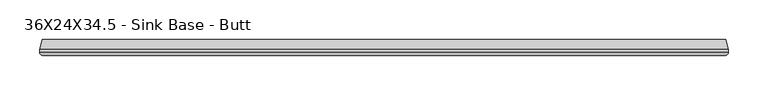
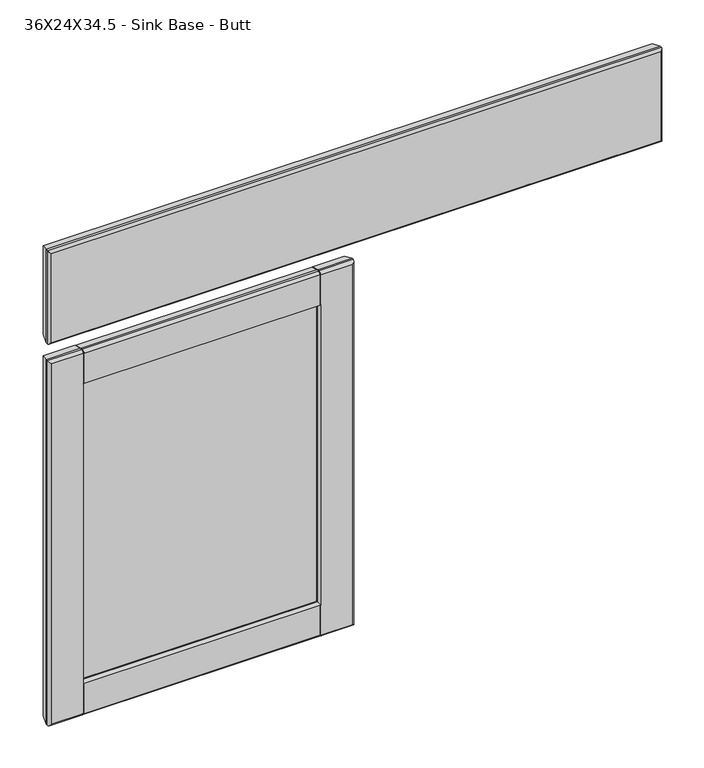
"""IFC4 building model written with IfcOpenShell, lengths in millimetres: furniture geometry, Cabinet-Base-Merillat-Double_Door-Marlin : 36X24X34.5 - Sink Base - Butt."""

from ifc_helpers import new_model, si_unit, frame, origin, place, context, project, spatial, polyline, circle_curve, ellipse_curve, outline, extrude, source, transform, mapped, element, save
from ifc_brep_helpers import plane_surface, cylinder_surface, advanced_brep


def furniture_36x24x34_5_sink_base_butt_1b95edc5(model_context):
    return source(origin(), model_context, "Body", "SolidModel", [
        advanced_brep(
        [(-413.1408026, -629.92, 847.8035075), (-413.1408026, -629.92, 714.2964925), (450.6162124, -629.92, 714.2964925), (450.6162124, -629.92, 847.8035075), (-412.7320951, -609.6, 714.7052), (-412.7320951, -609.6, 847.3948), (450.2075049, -609.6, 847.3948), (450.2075049, -609.6, 714.7052), (-416.2372951, -625.4496, 850.9), (-416.2372951, -622.681, 850.9), (-416.2372951, -622.681, 711.2), (-416.2372951, -625.4496, 711.2), (453.7127049, -622.681, 711.2), (453.7127049, -625.4496, 711.2), (453.7127049, -622.681, 850.9), (453.7127049, -625.4496, 850.9)],
        [
            (0, 1),
            (1, 2),
            (2, 3),
            (3, 0),
            (4, 5),
            (5, 6),
            (6, 7),
            (7, 4),
            (8, 9),
            (9, 10),
            (10, 11),
            (11, 8),
            (10, 12),
            (12, 13),
            (13, 11),
            (12, 14),
            (14, 15),
            (15, 13),
            (8, 15),
            (14, 9),
            (11, 1, ellipse_curve(frame((-411.4620951, -625.4496, 715.9752), z_axis=(-0.7071067811865475, 0.0, 0.7071067811865475), x_axis=(-0.7071067811865474, 0.0, -0.7071067811865476)), 6.7531526, 4.7752)),
            (0, 8, ellipse_curve(frame((-411.4620951, -625.4496, 846.1248), z_axis=(-0.7071067811865475, 0.0, -0.7071067811865475), x_axis=(0.7071067811865474, 0.0, -0.7071067811865476)), 6.7531526, 4.7752)),
            (4, 10),
            (9, 5),
            (13, 2, ellipse_curve(frame((448.9375049, -625.4496, 715.9752), z_axis=(-0.7071067811865475, 0.0, -0.7071067811865475), x_axis=(0.7071067811865476, 0.0, -0.7071067811865474)), 6.7531526, 4.7752)),
            (7, 12),
            (15, 3, ellipse_curve(frame((448.9375049, -625.4496, 846.1248), z_axis=(0.7071067811865475, 0.0, -0.7071067811865475), x_axis=(0.7071067811865474, 0.0, 0.7071067811865476)), 6.7531526, 4.7752)),
            (6, 14),
        ],
        [
            plane_surface(frame((-416.2372951, -629.92, 850.9), z_axis=(0.0, -1.0, 0.0), x_axis=(0.0, 0.0, -1.0))),
            plane_surface(frame((-416.2372951, -609.6, 850.9), z_axis=(0.0, 1.0, 0.0), x_axis=(0.0, 0.0, 1.0))),
            plane_surface(frame((-416.2372951, -629.92, 850.9), z_axis=(-1.0, 0.0, 0.0), x_axis=(0.0, 1.0, 0.0))),
            plane_surface(frame((-416.2372951, -629.92, 711.2), z_axis=(0.0, 0.0, -1.0), x_axis=(0.0, 1.0, 0.0))),
            plane_surface(frame((453.7127049, -629.92, 711.2), z_axis=(1.0, 0.0, 0.0), x_axis=(0.0, 1.0, 0.0))),
            plane_surface(frame((453.7127049, -629.92, 850.9), z_axis=(0.0, 0.0, 1.0), x_axis=(0.0, 1.0, 0.0))),
            cylinder_surface(frame((-411.4620951, -625.4496, 850.9), z_axis=(0.0, 0.0, -1.0), x_axis=(0.0, 1.0, 0.0)), 4.7752),
            plane_surface(frame((-416.2372951, -622.681, 850.9), z_axis=(-0.9659229350723619, 0.25882983502910506, 0.0), x_axis=(0.0, 0.0, -1.0))),
            cylinder_surface(frame((-416.2372951, -625.4496, 715.9752), z_axis=(1.0, 0.0, 0.0), x_axis=(0.0, 1.0, 0.0)), 4.7752),
            plane_surface(frame((-416.2372951, -622.681, 711.2), z_axis=(0.0, 0.25882983502910506, -0.9659229350723619), x_axis=(1.0, 0.0, 0.0))),
            cylinder_surface(frame((448.9375049, -625.4496, 711.2), z_axis=(0.0, 0.0, 1.0), x_axis=(0.0, 1.0, 0.0)), 4.7752),
            plane_surface(frame((453.7127049, -622.681, 711.2), z_axis=(0.9659229350723619, 0.25882983502910506, 0.0), x_axis=(0.0, 0.0, 1.0))),
            cylinder_surface(frame((453.7127049, -625.4496, 846.1248), z_axis=(-1.0, 0.0, 0.0), x_axis=(0.0, 1.0, 0.0)), 4.7752),
            plane_surface(frame((453.7127049, -622.681, 850.9), z_axis=(0.0, 0.25882983502910506, 0.9659229350723619), x_axis=(-1.0, 0.0, 0.0))),
        ],
        [
            (0, [[1, 2, 3, 4]]),
            (1, [[5, 6, 7, 8]]),
            (2, [[9, 10, 11, 12]]),
            (3, [[-11, 13, 14, 15]]),
            (4, [[-14, 16, 17, 18]]),
            (5, [[-9, 19, -17, 20]]),
            (6, [[21, -1, 22, -12]]),
            (7, [[23, -10, 24, -5]]),
            (8, [[-21, -15, 25, -2]]),
            (9, [[-23, -8, 26, -13]]),
            (10, [[-25, -18, 27, -3]]),
            (11, [[-26, -7, 28, -16]]),
            (12, [[-22, -4, -27, -19]]),
            (13, [[-24, -20, -28, -6]]),
        ],
    ),
        advanced_brep(
        [(-416.2372951, -625.4496, 685.8), (-416.2372951, -625.4496, 139.7), (-413.1408026, -629.92, 142.7964925), (-413.1408026, -629.92, 682.7035075), (-416.2372951, -622.681, 685.8), (-416.2372951, -622.681, 139.7), (-412.7320951, -609.6, 682.2948), (-412.7320951, -609.6, 143.2052), (-368.0361323, -609.6, 637.5988372), (-367.6660006, -610.39375, 637.2287055), (-365.5848416, -614.85681, 635.1475465), (-365.5848416, -614.85681, 190.3524535), (-367.6660006, -610.39375, 188.2712945), (-368.0361323, -609.6, 187.9011628), (-366.984611, -617.0969093, 636.547316), (-366.984611, -617.0969093, 188.952684), (-381.3122951, -617.347, 650.875), (-381.3122951, -617.347, 174.625), (-381.3122951, -622.173, 650.875), (-381.3122951, -622.173, 174.625), (-366.984611, -622.4230907, 636.547316), (-366.984611, -622.4230907, 188.952684), (-365.5848416, -624.66319, 635.1475465), (-365.5848416, -624.66319, 190.3524535), (-367.6660006, -629.12625, 637.2287055), (-368.0332649, -629.9138508, 637.5959698), (-368.0361323, -629.92, 187.9011628), (-367.6660006, -629.12625, 188.2712945), (14.0537124, -629.92, 142.7964925), (-31.0140137, -629.92, 142.7964925), (-31.0140137, -625.4496, 139.7), (17.1502049, -625.4496, 139.7), (-368.0332649, -625.4496, 139.7), (-368.0332649, -629.92, 142.7964925), (-366.4457649, -625.4496, 139.7), (-32.6015137, -625.4496, 139.7), (-32.6015137, -629.92, 142.7964925), (-366.4457649, -629.92, 142.7964925), (-31.0140137, -622.681, 139.7), (17.1502049, -622.681, 139.7), (-368.0332649, -622.681, 139.7), (-366.4457649, -622.681, 139.7), (-32.6015137, -622.681, 139.7), (-31.0140137, -609.6, 143.2052), (13.6450049, -609.6, 143.2052), (-366.4457649, -609.6, 143.2052), (-32.6015137, -609.6, 143.2052), (-368.0332649, -609.6, 143.2052), (-33.5022486, -614.85681, 190.3524535), (-31.4210895, -610.39375, 188.2712945), (-32.6015137, -610.39375, 188.2712945), (-32.6015137, -609.6, 187.9011628), (-366.4457649, -609.6, 187.9011628), (-366.4457649, -610.39375, 188.2712945), (-32.1024791, -617.0969093, 188.952684), (-17.7747951, -617.347, 174.625), (-17.7747951, -622.173, 174.625), (-32.1024791, -622.4230907, 188.952684), (-33.5022486, -624.66319, 190.3524535), (-366.4457649, -629.12625, 188.2712945), (-366.4457649, -629.92, 187.9011628), (-32.6015137, -629.92, 187.9011628), (-32.6015137, -629.12625, 188.2712945), (-31.4210895, -629.12625, 188.2712945), (17.1502049, -625.4496, 685.8), (14.0537124, -629.92, 682.7035075), (17.1502049, -622.681, 685.8), (13.6450049, -609.6, 682.2948), (-31.0509578, -609.6, 187.9011628), (-33.5022486, -614.85681, 635.1475465), (-31.4210895, -610.39375, 637.2287055), (-31.0509578, -609.6, 637.5988372), (-32.1024791, -617.0969093, 636.547316), (-17.7747951, -617.347, 650.875), (-17.7747951, -622.173, 650.875), (-32.1024791, -622.4230907, 636.547316), (-33.5022486, -624.66319, 635.1475465), (-31.0509578, -629.92, 187.9011628), (-31.0509578, -629.92, 637.5988372), (-31.4210895, -629.12625, 637.2287055), (-368.0332649, -629.92, 682.7035075), (-368.0332649, -625.4496, 685.8), (-31.0140137, -625.4496, 685.8), (-31.0140137, -629.92, 682.7035075), (-32.6015137, -625.4496, 685.8), (-366.4457649, -625.4496, 685.8), (-366.4457649, -629.92, 682.7035075), (-32.6015137, -629.92, 682.7035075), (-368.0332649, -622.681, 685.8), (-31.0140137, -622.681, 685.8), (-32.6015137, -622.681, 685.8), (-366.4457649, -622.681, 685.8), (-368.0332649, -609.6, 682.2948), (-31.0140137, -609.6, 682.2948), (-32.6015137, -609.6, 682.2948), (-366.4457649, -609.6, 682.2948), (-32.6015137, -609.6, 637.5988372), (-366.4457649, -609.6, 637.5988372), (-366.4457649, -610.39375, 637.2287055), (-32.6015137, -610.39375, 637.2287055), (-32.6015137, -629.12625, 637.2287055), (-32.6015137, -629.92, 637.5988372), (-366.4457649, -629.92, 637.5988372), (-366.4457649, -629.12625, 637.2287055), (-32.6015137, -629.12625, 682.5526052), (-32.6015137, -625.4496, 685.00625), (-32.6015137, -622.7855037, 685.00625), (-32.6015137, -610.39375, 681.6857412), (-31.0140137, -610.39375, 637.2287055), (-31.0140137, -610.39375, 681.6857412), (-31.0140137, -622.7855037, 685.00625), (-31.0140137, -625.4496, 685.00625), (-31.0140137, -629.12625, 682.5526052), (-31.0140137, -629.12625, 637.2287055), (-368.0332649, -629.12625, 637.2287055), (-368.0332649, -629.12625, 682.5526052), (-368.0332649, -625.4496, 685.00625), (-368.0332649, -622.7855037, 685.00625), (-368.0332649, -610.39375, 681.6857412), (-368.0332649, -610.39375, 637.2287055), (-366.4457649, -610.39375, 681.6857412), (-366.4457649, -622.7855037, 685.00625), (-366.4457649, -625.4496, 685.00625), (-366.4457649, -629.12625, 682.5526052), (-368.0332649, -610.39375, 188.2712945), (-368.0332649, -610.39375, 143.8142588), (-368.0332649, -622.7855037, 140.49375), (-368.0332649, -625.4496, 140.49375), (-368.0332649, -629.12625, 142.9473948), (-368.0332649, -629.12625, 188.2712945), (-366.4457649, -629.12625, 142.9473948), (-366.4457649, -625.4496, 140.49375), (-366.4457649, -622.7855037, 140.49375), (-366.4457649, -610.39375, 143.8142588), (-32.6015137, -610.39375, 143.8142588), (-32.6015137, -622.7855037, 140.49375), (-32.6015137, -625.4496, 140.49375), (-32.6015137, -629.12625, 142.9473948), (-31.0140137, -629.12625, 188.2712945), (-31.0140137, -629.12625, 142.9473948), (-31.0140137, -625.4496, 140.49375), (-31.0140137, -622.7855037, 140.49375), (-31.0140137, -610.39375, 143.8142588), (-31.0140137, -610.39375, 188.2712945)],
        [
            (0, 1),
            (1, 2, ellipse_curve(frame((-411.4620951, -625.4496, 144.4752), z_axis=(-0.7071067811865475, 0.0, 0.7071067811865475), x_axis=(0.7071067811865474, 0.0, 0.7071067811865476)), 6.7531526, 4.7752)),
            (2, 3),
            (3, 0, ellipse_curve(frame((-411.4620951, -625.4496, 681.0248), z_axis=(-0.7071067811865475, 0.0, -0.7071067811865475), x_axis=(-0.7071067811865474, 0.0, 0.7071067811865476)), 6.7531526, 4.7752)),
            (0, 4),
            (4, 5),
            (5, 1),
            (4, 6),
            (6, 7),
            (7, 5),
            (8, 9),
            (9, 10),
            (10, 11),
            (11, 12),
            (12, 13),
            (13, 8),
            (10, 14, ellipse_curve(frame((-367.0120951, -615.5223492, 636.5748), z_axis=(-0.7071067811865475, 0.0, -0.7071067811865475), x_axis=(-0.7071067811865474, 0.0, 0.7071067811865476)), 2.2271035, 1.5748)),
            (14, 15),
            (15, 11, ellipse_curve(frame((-367.0120951, -615.5223492, 188.9252), z_axis=(-0.7071067811865475, 0.0, 0.7071067811865475), x_axis=(0.7071067811865474, 0.0, 0.7071067811865476)), 2.2271035, 1.5748)),
            (14, 16),
            (16, 17),
            (17, 15),
            (16, 18),
            (18, 19),
            (19, 17),
            (18, 20),
            (20, 21),
            (21, 19),
            (20, 22, ellipse_curve(frame((-367.0120951, -623.9976508, 636.5748), z_axis=(-0.7071067811865475, 0.0, -0.7071067811865475), x_axis=(-0.7071067811865474, 0.0, 0.7071067811865476)), 2.2271035, 1.5748)),
            (22, 23),
            (23, 21, ellipse_curve(frame((-367.0120951, -623.9976508, 188.9252), z_axis=(-0.7071067811865475, 0.0, 0.7071067811865475), x_axis=(0.7071067811865474, 0.0, 0.7071067811865476)), 2.2271035, 1.5748)),
            (22, 24),
            (24, 25),
            (25, 26),
            (26, 27),
            (27, 23),
            (28, 29),
            (29, 30, circle_curve(frame((-31.0140137, -625.4496, 144.4752), z_axis=(1.0, 0.0, 0.0), x_axis=(0.0, 1.0, 0.0)), 4.7752)),
            (30, 31),
            (31, 28, ellipse_curve(frame((12.3750049, -625.4496, 144.4752), z_axis=(-0.7071067811865475, 0.0, -0.7071067811865475), x_axis=(-0.7071067811865476, 0.0, 0.7071067811865474)), 6.7531526, 4.7752)),
            (1, 32),
            (32, 33, circle_curve(frame((-368.0332649, -625.4496, 144.4752), z_axis=(-1.0, 0.0, 0.0), x_axis=(0.0, 1.0, 0.0)), 4.7752)),
            (33, 2),
            (34, 35),
            (35, 36, circle_curve(frame((-32.6015137, -625.4496, 144.4752), z_axis=(-1.0, 0.0, 0.0), x_axis=(0.0, 1.0, 0.0)), 4.7752)),
            (36, 37),
            (37, 34, circle_curve(frame((-366.4457649, -625.4496, 144.4752), z_axis=(1.0, 0.0, 0.0), x_axis=(0.0, 1.0, 0.0)), 4.7752)),
            (30, 38),
            (38, 39),
            (39, 31),
            (5, 40),
            (40, 32),
            (41, 42),
            (42, 35),
            (34, 41),
            (38, 43),
            (43, 44),
            (44, 39),
            (45, 46),
            (46, 42),
            (41, 45),
            (7, 47),
            (47, 40),
            (48, 49),
            (49, 50),
            (50, 51),
            (51, 52),
            (52, 53),
            (53, 12),
            (11, 48),
            (15, 54),
            (54, 48, ellipse_curve(frame((-32.0749951, -615.5223492, 188.9252), z_axis=(-0.7071067811865475, 0.0, -0.7071067811865475), x_axis=(-0.7071067811865476, 0.0, 0.7071067811865474)), 2.2271035, 1.5748)),
            (17, 55),
            (55, 54),
            (19, 56),
            (56, 55),
            (21, 57),
            (57, 56),
            (23, 58),
            (58, 57, ellipse_curve(frame((-32.0749951, -623.9976508, 188.9252), z_axis=(-0.7071067811865475, 0.0, -0.7071067811865475), x_axis=(-0.7071067811865476, 0.0, 0.7071067811865474)), 2.2271035, 1.5748)),
            (27, 59),
            (59, 60),
            (60, 61),
            (61, 62),
            (62, 63),
            (63, 58),
            (31, 64),
            (64, 65, ellipse_curve(frame((12.3750049, -625.4496, 681.0248), z_axis=(0.7071067811865475, 0.0, -0.7071067811865475), x_axis=(-0.7071067811865474, 0.0, -0.7071067811865476)), 6.7531526, 4.7752)),
            (65, 28),
            (39, 66),
            (66, 64),
            (44, 67),
            (67, 66),
            (68, 49),
            (48, 69),
            (69, 70),
            (70, 71),
            (71, 68),
            (54, 72),
            (72, 69, ellipse_curve(frame((-32.0749951, -615.5223492, 636.5748), z_axis=(0.7071067811865475, 0.0, -0.7071067811865475), x_axis=(-0.7071067811865474, 0.0, -0.7071067811865476)), 2.2271035, 1.5748)),
            (55, 73),
            (73, 72),
            (56, 74),
            (74, 73),
            (57, 75),
            (75, 74),
            (58, 76),
            (76, 75, ellipse_curve(frame((-32.0749951, -623.9976508, 636.5748), z_axis=(0.7071067811865475, 0.0, -0.7071067811865475), x_axis=(-0.7071067811865474, 0.0, -0.7071067811865476)), 2.2271035, 1.5748)),
            (63, 77),
            (77, 78),
            (78, 79),
            (79, 76),
            (3, 80),
            (80, 81, circle_curve(frame((-368.0332649, -625.4496, 681.0248), z_axis=(-1.0, 0.0, 0.0), x_axis=(0.0, 1.0, 0.0)), 4.7752)),
            (81, 0),
            (64, 82),
            (82, 83, circle_curve(frame((-31.0140137, -625.4496, 681.0248), z_axis=(1.0, 0.0, 0.0), x_axis=(0.0, 1.0, 0.0)), 4.7752)),
            (83, 65),
            (84, 85),
            (85, 86, circle_curve(frame((-366.4457649, -625.4496, 681.0248), z_axis=(1.0, 0.0, 0.0), x_axis=(0.0, 1.0, 0.0)), 4.7752)),
            (86, 87),
            (87, 84, circle_curve(frame((-32.6015137, -625.4496, 681.0248), z_axis=(-1.0, 0.0, 0.0), x_axis=(0.0, 1.0, 0.0)), 4.7752)),
            (81, 88),
            (88, 4),
            (66, 89),
            (89, 82),
            (90, 91),
            (91, 85),
            (84, 90),
            (88, 92),
            (92, 6),
            (67, 93),
            (93, 89),
            (94, 95),
            (95, 91),
            (90, 94),
            (51, 46),
            (45, 52),
            (43, 68),
            (71, 93),
            (92, 8),
            (13, 47),
            (96, 97),
            (97, 95),
            (94, 96),
            (9, 98),
            (98, 97),
            (96, 99),
            (99, 70),
            (69, 10),
            (72, 14),
            (73, 16),
            (74, 18),
            (75, 20),
            (76, 22),
            (79, 100),
            (100, 101),
            (101, 102),
            (102, 103),
            (103, 24),
            (33, 26),
            (25, 80),
            (36, 61),
            (60, 37),
            (83, 78),
            (77, 29),
            (86, 102),
            (101, 87),
            (100, 104),
            (104, 105, circle_curve(frame((-32.6015137, -625.4496, 681.0248), z_axis=(-1.0, 0.0, 0.0), x_axis=(0.0, 0.0, 1.0)), 3.98145)),
            (105, 106),
            (106, 107),
            (107, 99),
            (71, 108),
            (108, 109),
            (109, 110),
            (110, 111),
            (111, 112, circle_curve(frame((-31.0140137, -625.4496, 681.0248), z_axis=(1.0, 0.0, 0.0), x_axis=(0.0, 0.0, 1.0)), 3.98145)),
            (112, 113),
            (113, 78),
            (113, 79),
            (112, 104),
            (111, 105),
            (110, 106),
            (109, 107),
            (108, 70),
            (25, 114),
            (114, 115),
            (115, 116, circle_curve(frame((-368.0332649, -625.4496, 681.0248), z_axis=(-1.0, 0.0, 0.0), x_axis=(0.0, 0.0, 1.0)), 3.98145)),
            (116, 117),
            (117, 118),
            (118, 119),
            (119, 8),
            (98, 120),
            (120, 121),
            (121, 122),
            (122, 123, circle_curve(frame((-366.4457649, -625.4496, 681.0248), z_axis=(1.0, 0.0, 0.0), x_axis=(0.0, 0.0, 1.0)), 3.98145)),
            (123, 103),
            (24, 114),
            (123, 115),
            (122, 116),
            (121, 117),
            (120, 118),
            (9, 119),
            (13, 124),
            (124, 125),
            (125, 126),
            (126, 127),
            (127, 128, circle_curve(frame((-368.0332649, -625.4496, 144.4752), z_axis=(-1.0, 0.0, 0.0), x_axis=(0.0, 0.0, 1.0)), 3.98145)),
            (128, 129),
            (129, 26),
            (59, 130),
            (130, 131, circle_curve(frame((-366.4457649, -625.4496, 144.4752), z_axis=(1.0, 0.0, 0.0), x_axis=(0.0, 0.0, 1.0)), 3.98145)),
            (131, 132),
            (132, 133),
            (133, 53),
            (12, 124),
            (133, 125),
            (132, 126),
            (131, 127),
            (130, 128),
            (27, 129),
            (50, 134),
            (134, 135),
            (135, 136),
            (136, 137, circle_curve(frame((-32.6015137, -625.4496, 144.4752), z_axis=(-1.0, 0.0, 0.0), x_axis=(0.0, 0.0, 1.0)), 3.98145)),
            (137, 62),
            (138, 139),
            (139, 140, circle_curve(frame((-31.0140137, -625.4496, 144.4752), z_axis=(1.0, 0.0, 0.0), x_axis=(0.0, 0.0, 1.0)), 3.98145)),
            (140, 141),
            (141, 142),
            (142, 143),
            (143, 68),
            (77, 138),
            (63, 138),
            (143, 49),
            (142, 134),
            (141, 135),
            (140, 136),
            (139, 137),
        ],
        [
            cylinder_surface(frame((-411.4620951, -625.4496, 685.8), z_axis=(0.0, 0.0, 1.0), x_axis=(0.0, 1.0, 0.0)), 4.7752),
            plane_surface(frame((-416.2372951, -625.4496, 685.8), z_axis=(-1.0, 0.0, 0.0), x_axis=(0.0, 0.0, -1.0))),
            plane_surface(frame((-416.2372951, -622.681, 685.8), z_axis=(-0.9659229350723619, 0.25882983502910506, 0.0), x_axis=(0.0, 0.0, -1.0))),
            plane_surface(frame((-368.0361323, -609.6, 637.5988372), z_axis=(0.9063077870366099, 0.4226182617407856, 0.0), x_axis=(0.0, 0.0, -1.0))),
            cylinder_surface(frame((-367.0120951, -615.5223492, 685.8), z_axis=(0.0, 0.0, 1.0000000000000002), x_axis=(0.01745240643729364, -0.9998476951563912, 0.0)), 1.5748),
            plane_surface(frame((-366.984611, -617.0969093, 636.547316), z_axis=(0.017452406437322144, -0.9998476951563906, 0.0), x_axis=(0.0, 0.0, -1.0))),
            plane_surface(frame((-381.3122951, -617.347, 650.875), z_axis=(1.0, 0.0, 0.0), x_axis=(0.0, 0.0, -1.0))),
            plane_surface(frame((-381.3122951, -622.173, 650.875), z_axis=(0.01745240643727848, 0.9998476951563914, 0.0), x_axis=(0.0, 0.0, -1.0))),
            cylinder_surface(frame((-367.0120951, -623.9976508, 685.8), z_axis=(0.0, 0.0, 1.0000000000000002), x_axis=(0.9063077870367326, -0.42261826174052236, 0.0)), 1.5748),
            plane_surface(frame((-365.5848416, -624.66319, 635.1475465), z_axis=(0.9063077870366333, -0.4226182617407352, 0.0), x_axis=(0.0, 0.0, -1.0))),
            cylinder_surface(frame((-416.2372951, -625.4496, 144.4752), z_axis=(-1.0, 0.0, 0.0), x_axis=(0.0, 1.0, 0.0)), 4.7752),
            plane_surface(frame((-416.2372951, -625.4496, 139.7), z_axis=(0.0, 0.0, -1.0), x_axis=(1.0, 0.0, 0.0))),
            plane_surface(frame((-416.2372951, -622.681, 139.7), z_axis=(0.0, 0.25882983502910506, -0.9659229350723619), x_axis=(1.0, 0.0, 0.0))),
            plane_surface(frame((-368.0361323, -609.6, 187.9011628), z_axis=(0.0, 0.4226182617407856, 0.9063077870366099), x_axis=(1.0, 0.0, 0.0))),
            cylinder_surface(frame((-416.2372951, -615.5223492, 188.9252), z_axis=(-1.0000000000000002, 0.0, 0.0), x_axis=(0.0, -0.9998476951563912, 0.01745240643729364)), 1.5748),
            plane_surface(frame((-366.984611, -617.0969093, 188.952684), z_axis=(0.0, -0.9998476951563906, 0.017452406437322144), x_axis=(1.0, 0.0, 0.0))),
            plane_surface(frame((-381.3122951, -617.347, 174.625), z_axis=(0.0, 0.0, 1.0), x_axis=(1.0, 0.0, 0.0))),
            plane_surface(frame((-381.3122951, -622.173, 174.625), z_axis=(0.0, 0.9998476951563914, 0.01745240643727848), x_axis=(1.0, 0.0, 0.0))),
            cylinder_surface(frame((-416.2372951, -623.9976508, 188.9252), z_axis=(-1.0000000000000002, 0.0, 0.0), x_axis=(0.0, -0.42261826174052236, 0.9063077870367326)), 1.5748),
            plane_surface(frame((-365.5848416, -624.66319, 190.3524535), z_axis=(0.0, -0.4226182617407352, 0.9063077870366333), x_axis=(1.0, 0.0, 0.0))),
            cylinder_surface(frame((12.3750049, -625.4496, 139.7), z_axis=(0.0, 0.0, -1.0), x_axis=(0.0, 1.0, 0.0)), 4.7752),
            plane_surface(frame((17.1502049, -625.4496, 139.7), z_axis=(1.0, 0.0, 0.0), x_axis=(0.0, 0.0, 1.0))),
            plane_surface(frame((17.1502049, -622.681, 139.7), z_axis=(0.9659229350723619, 0.25882983502910506, 0.0), x_axis=(0.0, 0.0, 1.0))),
            plane_surface(frame((-31.0509578, -609.6, 187.9011628), z_axis=(-0.9063077870366099, 0.4226182617407856, 0.0), x_axis=(0.0, 0.0, 1.0))),
            cylinder_surface(frame((-32.0749951, -615.5223492, 139.7), z_axis=(0.0, 0.0, -1.0000000000000002), x_axis=(-0.01745240643729364, -0.9998476951563912, 0.0)), 1.5748),
            plane_surface(frame((-32.1024791, -617.0969093, 188.952684), z_axis=(-0.017452406437322144, -0.9998476951563906, 0.0), x_axis=(0.0, 0.0, 1.0))),
            plane_surface(frame((-17.7747951, -617.347, 174.625), z_axis=(-1.0, 0.0, 0.0), x_axis=(0.0, 0.0, 1.0))),
            plane_surface(frame((-17.7747951, -622.173, 174.625), z_axis=(-0.01745240643727848, 0.9998476951563914, 0.0), x_axis=(0.0, 0.0, 1.0))),
            cylinder_surface(frame((-32.0749951, -623.9976508, 139.7), z_axis=(0.0, 0.0, -1.0000000000000002), x_axis=(-0.9063077870367326, -0.42261826174052236, 0.0)), 1.5748),
            plane_surface(frame((-33.5022486, -624.66319, 190.3524535), z_axis=(-0.9063077870366333, -0.4226182617407352, 0.0), x_axis=(0.0, 0.0, 1.0))),
            cylinder_surface(frame((17.1502049, -625.4496, 681.0248), z_axis=(1.0, 0.0, 0.0), x_axis=(0.0, 1.0, 0.0)), 4.7752),
            plane_surface(frame((17.1502049, -625.4496, 685.8), z_axis=(0.0, 0.0, 1.0), x_axis=(-1.0, 0.0, 0.0))),
            plane_surface(frame((17.1502049, -622.681, 685.8), z_axis=(0.0, 0.25882983502910506, 0.9659229350723619), x_axis=(-1.0, 0.0, 0.0))),
            plane_surface(frame((13.6450049, -609.6, 682.2948), z_axis=(0.0, 1.0, 0.0), x_axis=(-1.0, 0.0, 0.0))),
            plane_surface(frame((-31.0509578, -609.6, 637.5988372), z_axis=(0.0, 0.4226182617407856, -0.9063077870366099), x_axis=(-1.0, 0.0, 0.0))),
            cylinder_surface(frame((17.1502049, -615.5223492, 636.5748), z_axis=(1.0000000000000002, 0.0, 0.0), x_axis=(0.0, -0.9998476951563912, -0.01745240643729364)), 1.5748),
            plane_surface(frame((-32.1024791, -617.0969093, 636.547316), z_axis=(0.0, -0.9998476951563906, -0.017452406437322144), x_axis=(-1.0, 0.0, 0.0))),
            plane_surface(frame((-17.7747951, -617.347, 650.875), z_axis=(0.0, 0.0, -1.0), x_axis=(-1.0, 0.0, 0.0))),
            plane_surface(frame((-17.7747951, -622.173, 650.875), z_axis=(0.0, 0.9998476951563914, -0.01745240643727848), x_axis=(-1.0, 0.0, 0.0))),
            cylinder_surface(frame((17.1502049, -623.9976508, 636.5748), z_axis=(1.0000000000000002, 0.0, 0.0), x_axis=(0.0, -0.42261826174052236, -0.9063077870367326)), 1.5748),
            plane_surface(frame((-33.5022486, -624.66319, 635.1475465), z_axis=(0.0, -0.4226182617407352, -0.9063077870366333), x_axis=(-1.0, 0.0, 0.0))),
            plane_surface(frame((-31.0509578, -629.92, 637.5988372), z_axis=(0.0, -1.0, 0.0), x_axis=(-1.0, 0.0, 0.0))),
            plane_surface(frame((-32.6015137, -629.92, 637.5988372), z_axis=(1.0, 0.0, 0.0), x_axis=(0.0, 0.906307787036771, -0.4226182617404399))),
            plane_surface(frame((-31.0140137, -629.92, 637.5988372), z_axis=(-1.0, 0.0, 0.0), x_axis=(0.0, -0.906307787036771, 0.4226182617404399))),
            plane_surface(frame((-32.6015137, -629.92, 637.5988372), z_axis=(0.0, 0.4226182617404399, 0.906307787036771), x_axis=(1.0, 0.0, 0.0))),
            plane_surface(frame((-32.6015137, -629.12625, 637.2287055), z_axis=(0.0, -1.0, 0.0), x_axis=(1.0, 0.0, 0.0))),
            cylinder_surface(frame((-31.0140137, -625.4496, 681.0248), z_axis=(1.0, 0.0, 0.0), x_axis=(0.0, 0.0, 1.0)), 3.98145),
            plane_surface(frame((-32.6015137, -625.4496, 685.00625), z_axis=(0.0, 0.0, 1.0), x_axis=(1.0, 0.0, 0.0))),
            plane_surface(frame((-32.6015137, -622.7855037, 685.00625), z_axis=(0.0, 0.25882983502913415, 0.9659229350723542), x_axis=(1.0, 0.0, 0.0))),
            plane_surface(frame((-32.6015137, -610.39375, 681.6857412), z_axis=(0.0, 1.0, 0.0), x_axis=(1.0, 0.0, 0.0))),
            plane_surface(frame((-32.6015137, -610.39375, 637.2287055), z_axis=(0.0, -0.4226182617405111, 0.9063077870367379), x_axis=(1.0, 0.0, 0.0))),
            plane_surface(frame((-368.0332649, -629.92, 637.5988372), z_axis=(1.0, 0.0, 0.0), x_axis=(0.0, 0.9063077870367783, -0.42261826174042444))),
            plane_surface(frame((-366.4457649, -629.92, 637.5988372), z_axis=(-1.0, 0.0, 0.0), x_axis=(0.0, -0.9063077870367783, 0.42261826174042444))),
            plane_surface(frame((-368.0332649, -629.92, 637.5988372), z_axis=(0.0, 0.42261826174042444, 0.9063077870367783), x_axis=(1.0, 0.0, 0.0))),
            plane_surface(frame((-368.0332649, -629.12625, 637.2287055), z_axis=(0.0, -1.0, 0.0), x_axis=(1.0, 0.0, 0.0))),
            cylinder_surface(frame((-366.4457649, -625.4496, 681.0248), z_axis=(1.0, 0.0, 0.0), x_axis=(0.0, 0.0, 1.0)), 3.98145),
            plane_surface(frame((-368.0332649, -625.4496, 685.00625), z_axis=(0.0, 0.0, 1.0), x_axis=(1.0, 0.0, 0.0))),
            plane_surface(frame((-368.0332649, -622.7855037, 685.00625), z_axis=(0.0, 0.25882983502911566, 0.965922935072359), x_axis=(1.0, 0.0, 0.0))),
            plane_surface(frame((-368.0332649, -610.39375, 681.6857412), z_axis=(0.0, 1.0, 0.0), x_axis=(1.0, 0.0, 0.0))),
            plane_surface(frame((-368.0332649, -610.39375, 637.2287055), z_axis=(0.0, -0.42261826174056427, 0.9063077870367131), x_axis=(1.0, 0.0, 0.0))),
            plane_surface(frame((-368.0332649, -625.4496, 149.2504), z_axis=(1.0, 0.0, 0.0), x_axis=(0.0, -1.0, 0.0))),
            plane_surface(frame((-366.4457649, -625.4496, 149.2504), z_axis=(-1.0, 0.0, 0.0), x_axis=(0.0, 1.0, 0.0))),
            plane_surface(frame((-368.0332649, -609.6, 187.9011628), z_axis=(0.0, -0.42261826173999295, -0.9063077870369795), x_axis=(1.0, 0.0, 0.0))),
            plane_surface(frame((-368.0332649, -610.39375, 188.2712945), z_axis=(0.0, 1.0, 0.0), x_axis=(1.0, 0.0, 0.0))),
            plane_surface(frame((-368.0332649, -610.39375, 143.8142588), z_axis=(0.0, 0.2588298350290845, -0.9659229350723675), x_axis=(1.0, 0.0, 0.0))),
            plane_surface(frame((-368.0332649, -622.7855037, 140.49375), z_axis=(0.0, 0.0, -1.0), x_axis=(1.0, 0.0, 0.0))),
            cylinder_surface(frame((-366.4457649, -625.4496, 144.4752), z_axis=(1.0, 0.0, 0.0), x_axis=(0.0, 0.0, 1.0)), 3.98145),
            plane_surface(frame((-368.0332649, -629.12625, 142.9473948), z_axis=(0.0, -1.0, 0.0), x_axis=(1.0, 0.0, 0.0))),
            plane_surface(frame((-368.0332649, -629.12625, 188.2712945), z_axis=(0.0, 0.4226182617407698, -0.9063077870366172), x_axis=(1.0, 0.0, 0.0))),
            plane_surface(frame((-32.6015137, -629.12625, 188.2712945), z_axis=(1.0, 0.0, 0.0), x_axis=(0.0, -0.906307787036583, -0.42261826174084305))),
            plane_surface(frame((-31.0140137, -629.12625, 188.2712945), z_axis=(-1.0, 0.0, 0.0), x_axis=(0.0, 0.906307787036583, 0.42261826174084305))),
            plane_surface(frame((-32.6015137, -629.12625, 188.2712945), z_axis=(0.0, 0.42261826174084305, -0.906307787036583), x_axis=(1.0, 0.0, 0.0))),
            plane_surface(frame((-32.6015137, -609.6, 187.9011628), z_axis=(0.0, -0.42261826174073325, -0.9063077870366342), x_axis=(1.0, 0.0, 0.0))),
            plane_surface(frame((-32.6015137, -610.39375, 188.2712945), z_axis=(0.0, 1.0, 0.0), x_axis=(1.0, 0.0, 0.0))),
            plane_surface(frame((-32.6015137, -610.39375, 143.8142588), z_axis=(0.0, 0.2588298350290967, -0.9659229350723642), x_axis=(1.0, 0.0, 0.0))),
            plane_surface(frame((-32.6015137, -622.7855037, 140.49375), z_axis=(0.0, 0.0, -1.0), x_axis=(1.0, 0.0, 0.0))),
            cylinder_surface(frame((-31.0140137, -625.4496, 144.4752), z_axis=(1.0, 0.0, 0.0), x_axis=(0.0, 0.0, 1.0)), 3.98145),
            plane_surface(frame((-32.6015137, -629.12625, 142.9473948), z_axis=(0.0, -1.0, 0.0), x_axis=(1.0, 0.0, 0.0))),
        ],
        [
            (0, [[1, 2, 3, 4]]),
            (1, [[5, 6, 7, -1]]),
            (2, [[8, 9, 10, -6]]),
            (3, [[11, 12, 13, 14, 15, 16]]),
            (4, [[17, 18, 19, -13]]),
            (5, [[20, 21, 22, -18]]),
            (6, [[23, 24, 25, -21]]),
            (7, [[26, 27, 28, -24]]),
            (8, [[29, 30, 31, -27]]),
            (9, [[32, 33, 34, 35, 36, -30]]),
            (10, [[37, 38, 39, 40]]),
            (10, [[41, 42, 43, -2]]),
            (10, [[44, 45, 46, 47]]),
            (11, [[-39, 48, 49, 50]]),
            (11, [[51, 52, -41, -7]]),
            (11, [[53, 54, -44, 55]]),
            (12, [[-49, 56, 57, 58]]),
            (12, [[59, 60, -53, 61]]),
            (12, [[62, 63, -51, -10]]),
            (13, [[64, 65, 66, 67, 68, 69, -14, 70]]),
            (14, [[71, 72, -70, -19]]),
            (15, [[73, 74, -71, -22]]),
            (16, [[75, 76, -73, -25]]),
            (17, [[77, 78, -75, -28]]),
            (18, [[79, 80, -77, -31]]),
            (19, [[-36, 81, 82, 83, 84, 85, 86, -79]]),
            (20, [[87, 88, 89, -40]]),
            (21, [[90, 91, -87, -50]]),
            (22, [[92, 93, -90, -58]]),
            (23, [[94, -64, 95, 96, 97, 98]]),
            (24, [[99, 100, -95, -72]]),
            (25, [[101, 102, -99, -74]]),
            (26, [[103, 104, -101, -76]]),
            (27, [[105, 106, -103, -78]]),
            (28, [[107, 108, -105, -80]]),
            (29, [[-86, 109, 110, 111, 112, -107]]),
            (30, [[113, 114, 115, -4]]),
            (30, [[116, 117, 118, -88]]),
            (30, [[119, 120, 121, 122]]),
            (31, [[-115, 123, 124, -5]]),
            (31, [[125, 126, -116, -91]]),
            (31, [[127, 128, -119, 129]]),
            (32, [[-124, 130, 131, -8]]),
            (32, [[132, 133, -125, -93]]),
            (32, [[134, 135, -127, 136]]),
            (33, [[-67, 137, -59, 138]]),
            (33, [[-57, 139, -98, 140, -132, -92]]),
            (33, [[-131, 141, -16, 142, -62, -9]]),
            (33, [[143, 144, -134, 145]]),
            (34, [[-12, 146, 147, -143, 148, 149, -96, 150]]),
            (35, [[-150, -100, 151, -17]]),
            (36, [[-151, -102, 152, -20]]),
            (37, [[-152, -104, 153, -23]]),
            (38, [[-153, -106, 154, -26]]),
            (39, [[-154, -108, 155, -29]]),
            (40, [[-112, 156, 157, 158, 159, 160, -32, -155]]),
            (41, [[-43, 161, -34, 162, -113, -3]]),
            (41, [[-46, 163, -83, 164]]),
            (41, [[-118, 165, -110, 166, -37, -89]]),
            (41, [[-121, 167, -158, 168]]),
            (42, [[-148, -145, -136, -129, -122, -168, -157, 169, 170, 171, 172, 173]]),
            (43, [[-165, -117, -126, -133, -140, 174, 175, 176, 177, 178, 179, 180]]),
            (44, [[181, -111, -180]]),
            (45, [[-156, -181, -179, 182, -169]]),
            (46, [[-182, -178, 183, -170]]),
            (47, [[-183, -177, 184, -171]]),
            (48, [[-184, -176, 185, -172]]),
            (49, [[-185, -175, 186, -149, -173]]),
            (50, [[-97, -186, -174]]),
            (51, [[-141, -130, -123, -114, -162, 187, 188, 189, 190, 191, 192, 193]]),
            (52, [[-159, -167, -120, -128, -135, -144, -147, 194, 195, 196, 197, 198]]),
            (53, [[-33, 199, -187]]),
            (54, [[-199, -160, -198, 200, -188]]),
            (55, [[-200, -197, 201, -189]]),
            (56, [[-201, -196, 202, -190]]),
            (57, [[-202, -195, 203, -191]]),
            (58, [[-203, -194, -146, 204, -192]]),
            (59, [[-204, -11, -193]]),
            (60, [[-161, -42, -52, -63, -142, 205, 206, 207, 208, 209, 210, 211]]),
            (61, [[-68, -138, -61, -55, -47, -164, -82, 212, 213, 214, 215, 216]]),
            (62, [[-15, 217, -205]]),
            (63, [[-217, -69, -216, 218, -206]]),
            (64, [[-218, -215, 219, -207]]),
            (65, [[-219, -214, 220, -208]]),
            (66, [[-220, -213, 221, -209]]),
            (67, [[-221, -212, -81, 222, -210]]),
            (68, [[-222, -35, -211]]),
            (69, [[-84, -163, -45, -54, -60, -137, -66, 223, 224, 225, 226, 227]]),
            (70, [[228, 229, 230, 231, 232, 233, -139, -56, -48, -38, -166, 234]]),
            (71, [[-109, 235, -234]]),
            (72, [[236, -94, -233]]),
            (73, [[-65, -236, -232, 237, -223]]),
            (74, [[-237, -231, 238, -224]]),
            (75, [[-238, -230, 239, -225]]),
            (76, [[-239, -229, 240, -226]]),
            (77, [[-240, -228, -235, -85, -227]]),
        ],
    ),
        extrude(outline(polyline([(-17.7747951, -622.173), (-381.3122951, -622.173), (-381.3122951, -617.347), (-17.7747951, -617.347), (-17.7747951, -622.173)])), frame((0.0, 0.0, 174.625), z_axis=(0.0, 0.0, 1.0), x_axis=(1.0, 0.0, 0.0)), (0.0, 0.0, 1.0), 476.25),
    ])


if __name__ == "__main__":
    model = new_model("IFC4")
    model_context = context("Model", 3, world=origin())
    ifc_project = project(units=[si_unit("LENGTHUNIT", "METRE", prefix="MILLI")], contexts=[model_context])
    site = spatial("IfcSite", under=ifc_project)
    building = spatial("IfcBuilding", under=site)
    placement = place(None, origin())
    furniture_36x24x34_5_sink_base_butt_shape = furniture_36x24x34_5_sink_base_butt_1b95edc5(model_context)
    element("IfcFurniture", 1, ObjectType="Cabinet-Base-Merillat-Double_Door-Marlin : 36X24X34.5 - Sink Base - Butt", at=placement, inside=building, context=model_context, shape_type="MappedRepresentation", body=[
        mapped(furniture_36x24x34_5_sink_base_butt_shape, transform((0.0, 0.0, 0.0), x_axis=(1.0, 0.0, 0.0), y_axis=(0.0, 1.0, 0.0), z_axis=(0.0, 0.0, 1.0))),
    ])
    save(model, "model.ifc")

# Revit data of these elements
# Type "Cabinet-Base-Merillat-Double_Door-Marlin : 36X24X34.5 - Sink Base - Butt"
#   URL = "http://www.merillat.com"
#   Toe Kick Note = "Toe Kick Covering is not included. To be purchased Separately."
#   Product Line = "Express"
#   Product Page URL = "http://www.merillat.com//our-products/rooms/kitchen"
#   Product Group = "Base Cabinet"
#   Product Documentation Link = "http://merillatbusiness.com/customer-resources/product-line-resources/merillat-classic/"
#   Model = "SB36B"
#   Manufacturer = "Merillat"
#   Finish = "Wood"
#   Description = "Sink Base Double Door Butt"
#   Construction Type = "Deep Sink Base"
#   Cabinet Construction Note = "No shelf, One full width false drawer front above doors except SB42, SB4227 and SB48 which have two drawer fronts, Roll-out tray N/A for 27\" deep cabinets"
#   Assembly Code = "C1030410"
#   Toe Kick Height = 0' - 4 1/2"
#   Toe Kick Depth = 0' - 2 25/32"
#   Top and Bottom Spacing = 0' - 1"
#   Side Spacing = 0' - 0 7/8"
#   Cabinet Shell = 0' - 0 3/8"
#   Door Spacing = 0' - 0 1/8"
#   Depth = 2' - 0"
#   Height = 2' - 10 1/2"
#   Width = 3' - 0"
#   Cabinet Drawer Width = 2' - 10 1/4"
#   Cabinet Drawer Height = 0' - 5 1/2"
#   Cabinet Drawer 2 Drawer Width = 1' - 5 1/16"
#   Cabinet Door Width = 1' - 5 1/16"
#   Cabinet Door Height = 1' - 9 1/2"
#   COBie.Type = no
#   Two Drawer = no
#   Elevation Swing Line = yes
#   Partial Overlay = yes
#   One Drawer = yes
#   Full Overlay = no
#   Butt Option = yes
#   Toe Kick Material = Wood - Merillat - Raw Particle Board
#   Door Drawer Material = Wood - Merillat - Pecan(1)
#   Cabinet Material = Wood - Merillat - Pecan(1)
#   Cabinet Drawer Style 2 Drawer = element 819256
#   Cabinet Drawer Style = element 819255
#   Cabinet Door Style = element 819254
# Element 1 (IfcFurniture, "Cabinet-Base-Merillat-Double_Door-Marlin : 36X24X34.5 - Sink Base - Butt")
#   Materials on its faces: "Wood - Merillat - Pecan(1)", "Wood - Merillat - Raw Particle Board"
# Materials
#   "Wood - Merillat - Raw Particle Board": class "Plastic", colour RGB 80 80 80, transparency 0, Description = "Plastic Laminate - Navy", Cost = 0
#   "Wood - Merillat - Pecan(1)": class "Wood", colour RGB 108 67 43, transparency 0, Cost = 0
